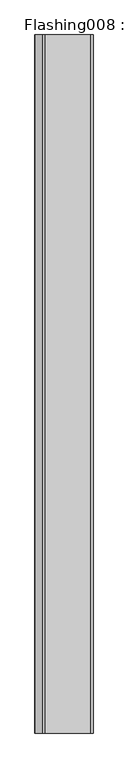
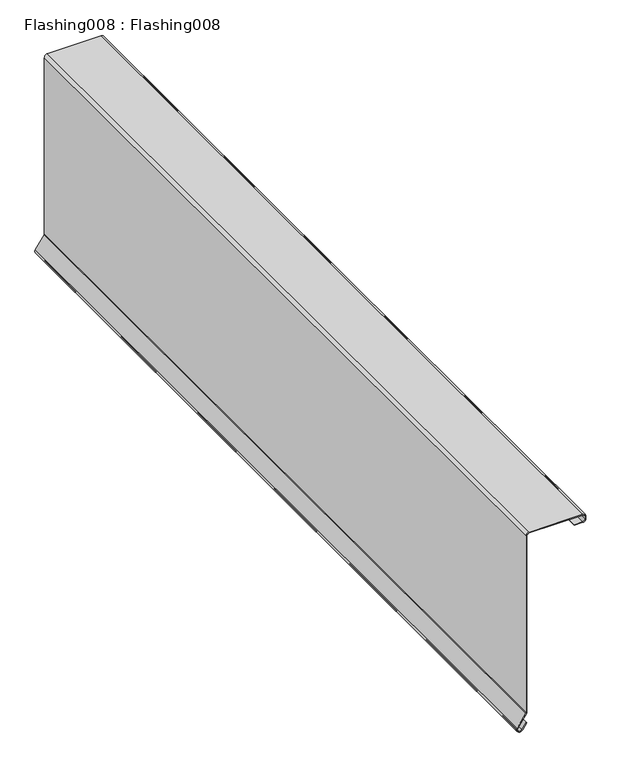
"""IFC4 building model written with IfcOpenShell, lengths in millimetres: proxy geometry, Flashing008 : Flashing008."""

from ifc_helpers import new_model, si_unit, point, frame, frame_2d, origin, place, context, project, spatial, polyline, circle_curve, trimmed, segment, composite_curve, outline, extrude, source, transform, mapped, element, save


def flashing008_flashing008_516c5e6e(model_context):
    return source(origin(), model_context, "Body", "SweptSolid", [
        extrude(outline(composite_curve([segment(trimmed(circle_curve(frame_2d((43033.8898747, -6514.9327408)), 5.08), [point((43030.9678143, -6510.7772669))], [point((43029.7783694, -6517.9163501))], True, "CARTESIAN"), True, "CONTINUOUS"), segment(polyline([(43029.7783694, -6517.9163501), (43031.0710485, -6519.6977016)]), True, "CONTINUOUS"), segment(trimmed(circle_curve(frame_2d((43035.1825538, -6516.7140923)), 5.08), [point((43031.0710485, -6519.6977016))], [point((43038.0896432, -6520.8800533))], True, "CARTESIAN"), True, "CONTINUOUS"), segment(polyline([(43038.0896432, -6520.8800533), (43068.3424938, -6499.7690195)]), True, "CONTINUOUS"), segment(trimmed(circle_curve(frame_2d((43071.2495833, -6503.9349805)), 5.08), [point((43068.3424938, -6499.7690195))], [point((43071.2495833, -6498.8549805))], False, "CARTESIAN"), True, "CONTINUOUS"), segment(polyline([(43071.2495833, -6498.8549805), (43518.4785937, -6498.8549805)]), True, "CONTINUOUS"), segment(trimmed(circle_curve(frame_2d((43518.4785937, -6493.7749805)), 5.08), [point((43518.4785937, -6498.8549805))], [point((43523.5585937, -6493.7749805))], True, "CARTESIAN"), True, "CONTINUOUS"), segment(polyline([(43523.5585937, -6493.7749805), (43523.5585937, -6364.4349805)]), True, "CONTINUOUS"), segment(trimmed(circle_curve(frame_2d((43518.4785937, -6364.4349805)), 5.08), [point((43523.5585937, -6364.4349805))], [point((43518.4785937, -6359.3549805))], True, "CARTESIAN"), True, "CONTINUOUS"), segment(polyline([(43518.4785937, -6359.3549805), (43512.0721875, -6359.3549805)]), True, "CONTINUOUS"), segment(trimmed(circle_curve(frame_2d((43512.0721875, -6364.4349805)), 5.08), [point((43512.0721875, -6359.3549805))], [point((43506.9921875, -6364.4349805))], True, "CARTESIAN"), True, "CONTINUOUS"), segment(polyline([(43506.9921875, -6364.4349805), (43506.9921875, -6385.7314453), (43504.9921875, -6385.7314453), (43504.9921875, -6364.4349805)]), True, "CONTINUOUS"), segment(trimmed(circle_curve(frame_2d((43512.0721875, -6364.4349805)), 7.08), [point((43504.9921875, -6364.4349805))], [point((43512.0721875, -6357.3549805))], False, "CARTESIAN"), True, "CONTINUOUS"), segment(polyline([(43512.0721875, -6357.3549805), (43518.4785937, -6357.3549805)]), True, "CONTINUOUS"), segment(trimmed(circle_curve(frame_2d((43518.4785937, -6364.4349805)), 7.08), [point((43518.4785937, -6357.3549805))], [point((43525.5585937, -6364.4349805))], False, "CARTESIAN"), True, "CONTINUOUS"), segment(polyline([(43525.5585937, -6364.4349805), (43525.5585937, -6493.7749805)]), True, "CONTINUOUS"), segment(trimmed(circle_curve(frame_2d((43518.4785937, -6493.7749805)), 7.08), [point((43525.5585937, -6493.7749805))], [point((43518.4785937, -6500.8549805))], False, "CARTESIAN"), True, "CONTINUOUS"), segment(polyline([(43518.4785937, -6500.8549805), (43071.2495833, -6500.8549805)]), True, "CONTINUOUS"), segment(trimmed(circle_curve(frame_2d((43071.2495833, -6503.9349805)), 3.08), [point((43071.2495833, -6500.8549805))], [point((43069.4870172, -6501.4091616))], True, "CARTESIAN"), True, "CONTINUOUS"), segment(polyline([(43069.4870172, -6501.4091616), (43039.2341666, -6522.5201954)]), True, "CONTINUOUS"), segment(trimmed(circle_curve(frame_2d((43035.1825538, -6516.7140923)), 7.08), [point((43039.2341666, -6522.5201954))], [point((43029.4523457, -6520.872351))], False, "CARTESIAN"), True, "CONTINUOUS"), segment(polyline([(43029.4523457, -6520.872351), (43028.1596666, -6519.0909995)]), True, "CONTINUOUS"), segment(trimmed(circle_curve(frame_2d((43033.8898747, -6514.9327408)), 7.08), [point((43028.1596666, -6519.0909995))], [point((43029.8173969, -6509.1412536))], False, "CARTESIAN"), True, "CONTINUOUS"), segment(polyline([(43029.8173969, -6509.1412536), (43044.40427, -6498.8840062), (43045.5546875, -6500.5200195), (43030.9678143, -6510.7772669)]), True, "CONTINUOUS")], self_intersect=False)), frame((0.0, 7982.1531721, 0.0), z_axis=(0.0, 1.0, 0.0), x_axis=(0.0, 0.0, 1.0)), (0.0, 0.0, 1.0), 2000.0),
    ])


if __name__ == "__main__":
    model = new_model("IFC4")
    model_context = context("Model", 3, world=origin())
    ifc_project = project(units=[si_unit("LENGTHUNIT", "METRE", prefix="MILLI")], contexts=[model_context])
    site = spatial("IfcSite", under=ifc_project)
    building = spatial("IfcBuilding", under=site)
    placement = place(None, origin())
    flashing008_flashing008_shape = flashing008_flashing008_516c5e6e(model_context)
    element("IfcBuildingElementProxy", 1, Name="Flashing008 : Flashing008", ObjectType="Flashing008 : Flashing008", at=placement, inside=building, context=model_context, shape_type="MappedRepresentation", body=[
        mapped(flashing008_flashing008_shape, transform((0.0, 0.0, 0.0), x_axis=(1.0, 0.0, 0.0), y_axis=(0.0, 1.0, 0.0), z_axis=(0.0, 0.0, 1.0))),
    ])
    save(model, "model.ifc")

# Revit data of these elements
# Type "Flashing008 : Flashing008"
#   NameOverride = "Flashing008"
# Element 1 (IfcBuildingElementProxy, "Flashing008 : Flashing008")
#   Materials on its faces: "HIGH EAVE FLASHING"
# Materials
#   "HIGH EAVE FLASHING": class "Unassigned", colour RGB 128 128 128, transparency 0
